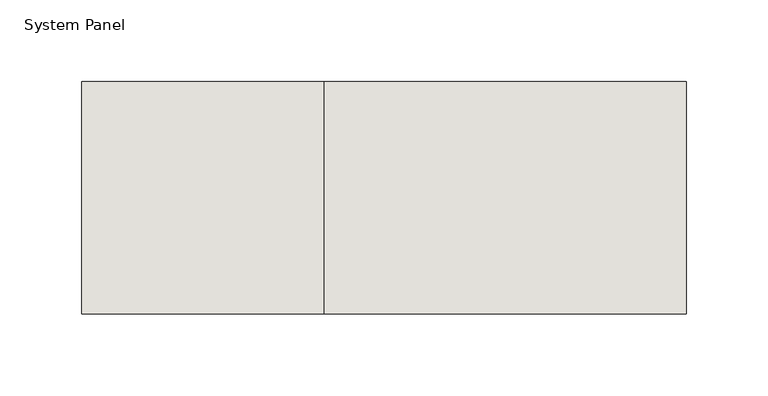
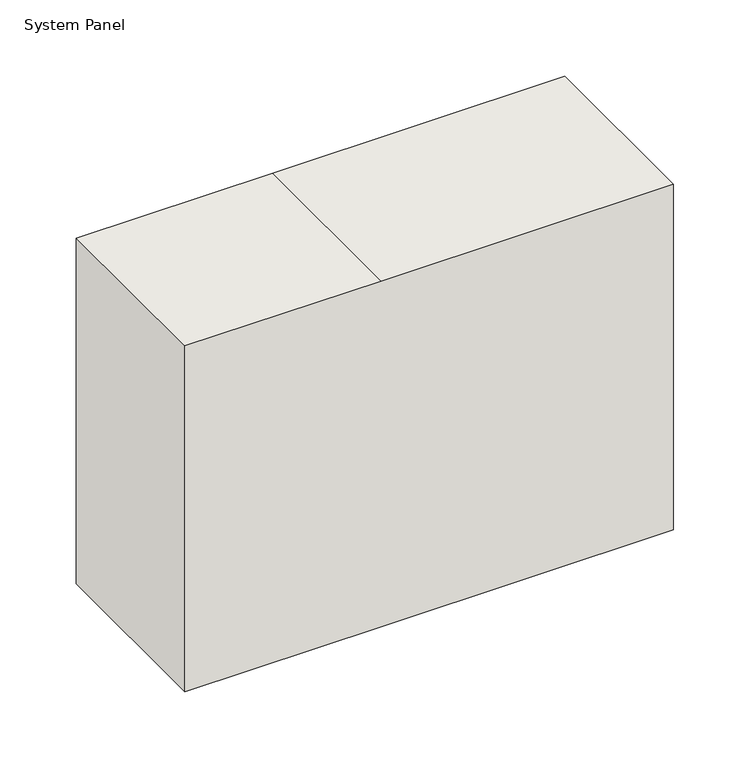
"""IFC4 building model written with IfcOpenShell, lengths in millimetres: wall geometry, System Panel : NLRS_21_CWP_hsb-vulling minerale wol 142 _gen_rsf."""

from ifc_helpers import new_model, si_unit, frame, origin, place, context, project, spatial, polyline, outline, extrude, source, transform, mapped, element, save


def system_panel_c31e55ff(model_context):
    return source(origin(), model_context, "Body", "SweptSolid", [
        extrude(outline(polyline([(0.0, -184.5), (0.0, -36.3441061), (0.0, 184.5), (276.0, 184.5), (276.0, -36.3441061), (276.0, -184.5), (0.0, -184.5)])), frame((0.0, -71.0, 0.0), z_axis=(0.0, 1.0, 0.0), x_axis=(0.0, 0.0, 1.0)), (0.0, 0.0, 1.0), 142.0),
    ])


if __name__ == "__main__":
    model = new_model("IFC4")
    model_context = context("Model", 3, world=origin())
    ifc_project = project(units=[si_unit("LENGTHUNIT", "METRE", prefix="MILLI")], contexts=[model_context])
    site = spatial("IfcSite", under=ifc_project)
    building = spatial("IfcBuilding", under=site)
    placement = place(None, origin())
    system_panel_shape = system_panel_c31e55ff(model_context)
    element("IfcWall", 1, ObjectType="System Panel : NLRS_21_CWP_hsb-vulling minerale wol 142 _gen_rsf", at=placement, inside=building, context=model_context, shape_type="MappedRepresentation", body=[
        mapped(system_panel_shape, transform((0.0, 0.0, 0.0), x_axis=(1.0, 0.0, 0.0), y_axis=(0.0, 1.0, 0.0), z_axis=(0.0, 0.0, 1.0))),
    ])
    save(model, "model.ifc")

# Revit data of these elements
# Type "System Panel : NLRS_21_CWP_hsb-vulling minerale wol 142 _gen_rsf"
#   Type IfcGUID = "07M7mRoiH1CR8m_RSKIwpC"
#   Assembly Code = "21.23"
#   IfcExportAs = "IfcWall"
# Element 1 (IfcWall, "System Panel : NLRS_21_CWP_hsb-vulling minerale wol 142 _gen_rsf")
#   Materials on its faces: "NLRS_m1_isolatie minerale wol_gen_rsf"
# Materials
#   "NLRS_m1_isolatie minerale wol_gen_rsf": class "M - Anorganische materialen", colour RGB 200 200 140, transparency 0, Keynote = "m1", Manufacturer = "Revit Standards Foundation", URL = "www.revitstandards.org", Description = "isolatie minerale wol", Cost = 0
